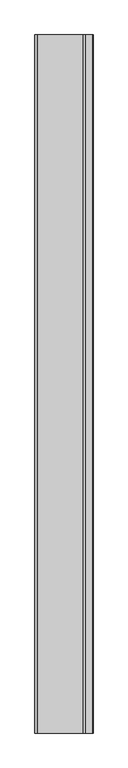
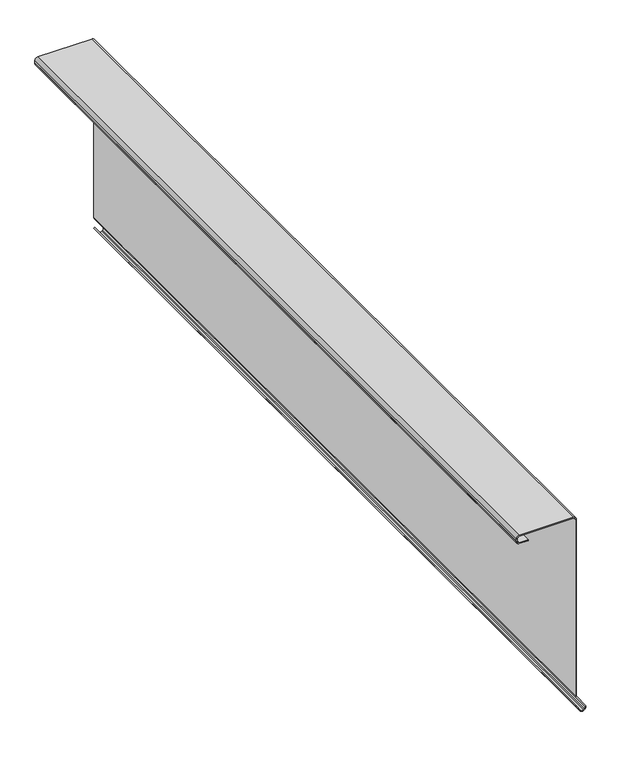
"""IFC4 building model written with IfcOpenShell, lengths in millimetres: proxy geometry, Flashing018 8742 : Flashing018 8742."""

from ifc_helpers import new_model, si_unit, point, frame, frame_2d, origin, place, context, project, spatial, polyline, circle_curve, trimmed, segment, composite_curve, outline, extrude, source, transform, mapped, element, save


def generic_models_9543aaf0(model_context):
    return source(origin(), model_context, "Body", "SweptSolid", [
        extrude(outline(composite_curve([segment(polyline([(43036.8907248, 17759.2743151), (43051.477598, 17749.0170677), (43050.3271805, 17747.3810543), (43035.7403074, 17757.6383018)]), True, "CONTINUOUS"), segment(trimmed(circle_curve(frame_2d((43039.8127852, 17763.429789)), 7.08), [point((43035.7403074, 17757.6383018))], [point((43034.0825771, 17767.5880476))], False, "CARTESIAN"), True, "CONTINUOUS"), segment(polyline([(43034.0825771, 17767.5880476), (43035.3752562, 17769.3693991)]), True, "CONTINUOUS"), segment(trimmed(circle_curve(frame_2d((43041.1054643, 17765.2111405)), 7.08), [point((43035.3752562, 17769.3693991))], [point((43045.1570771, 17771.0172436))], False, "CARTESIAN"), True, "CONTINUOUS"), segment(polyline([(43045.1570771, 17771.0172436), (43075.4099277, 17749.9062098)]), True, "CONTINUOUS"), segment(trimmed(circle_curve(frame_2d((43077.1724938, 17752.4320286)), 3.08), [point((43075.4099277, 17749.9062098))], [point((43077.1724938, 17749.3520286))], True, "CARTESIAN"), True, "CONTINUOUS"), segment(polyline([(43077.1724938, 17749.3520286), (43524.4015043, 17749.3520286)]), True, "CONTINUOUS"), segment(trimmed(circle_curve(frame_2d((43524.4015043, 17742.2720286)), 7.08), [point((43524.4015043, 17749.3520286))], [point((43531.4815043, 17742.2720286))], False, "CARTESIAN"), True, "CONTINUOUS"), segment(polyline([(43531.4815043, 17742.2720286), (43531.4815043, 17612.9320286)]), True, "CONTINUOUS"), segment(trimmed(circle_curve(frame_2d((43524.4015043, 17612.9320286)), 7.08), [point((43531.4815043, 17612.9320286))], [point((43524.4015043, 17605.8520286))], False, "CARTESIAN"), True, "CONTINUOUS"), segment(polyline([(43524.4015043, 17605.8520286), (43517.995098, 17605.8520286)]), True, "CONTINUOUS"), segment(trimmed(circle_curve(frame_2d((43517.995098, 17612.9320286)), 7.08), [point((43517.995098, 17605.8520286))], [point((43510.915098, 17612.9320286))], False, "CARTESIAN"), True, "CONTINUOUS"), segment(polyline([(43510.915098, 17612.9320286), (43510.915098, 17634.2284935), (43512.915098, 17634.2284935), (43512.915098, 17612.9320286)]), True, "CONTINUOUS"), segment(trimmed(circle_curve(frame_2d((43517.995098, 17612.9320286)), 5.08), [point((43512.915098, 17612.9320286))], [point((43517.995098, 17607.8520286))], True, "CARTESIAN"), True, "CONTINUOUS"), segment(polyline([(43517.995098, 17607.8520286), (43524.4015043, 17607.8520286)]), True, "CONTINUOUS"), segment(trimmed(circle_curve(frame_2d((43524.4015043, 17612.9320286)), 5.08), [point((43524.4015043, 17607.8520286))], [point((43529.4815043, 17612.9320286))], True, "CARTESIAN"), True, "CONTINUOUS"), segment(polyline([(43529.4815043, 17612.9320286), (43529.4815043, 17742.2720286)]), True, "CONTINUOUS"), segment(trimmed(circle_curve(frame_2d((43524.4015043, 17742.2720286)), 5.08), [point((43529.4815043, 17742.2720286))], [point((43524.4015043, 17747.3520286))], True, "CARTESIAN"), True, "CONTINUOUS"), segment(polyline([(43524.4015043, 17747.3520286), (43077.1724938, 17747.3520286)]), True, "CONTINUOUS"), segment(trimmed(circle_curve(frame_2d((43077.1724938, 17752.4320286)), 5.08), [point((43077.1724938, 17747.3520286))], [point((43074.2654043, 17748.2660676))], False, "CARTESIAN"), True, "CONTINUOUS"), segment(polyline([(43074.2654043, 17748.2660676), (43044.0125537, 17769.3771014)]), True, "CONTINUOUS"), segment(trimmed(circle_curve(frame_2d((43041.1054643, 17765.2111405)), 5.08), [point((43044.0125537, 17769.3771014))], [point((43036.993959, 17768.1947498))], True, "CARTESIAN"), True, "CONTINUOUS"), segment(polyline([(43036.993959, 17768.1947498), (43035.7012799, 17766.4133983)]), True, "CONTINUOUS"), segment(trimmed(circle_curve(frame_2d((43039.8127852, 17763.429789)), 5.08), [point((43035.7012799, 17766.4133983))], [point((43036.8907248, 17759.2743151))], True, "CARTESIAN"), True, "CONTINUOUS")], self_intersect=False)), frame((0.0, 7982.1507711, 0.0), z_axis=(0.0, 1.0, 0.0), x_axis=(0.0, 0.0, 1.0)), (0.0, 0.0, 1.0), 2000.0),
    ])


if __name__ == "__main__":
    model = new_model("IFC4")
    model_context = context("Model", 3, world=origin())
    ifc_project = project(units=[si_unit("LENGTHUNIT", "METRE", prefix="MILLI")], contexts=[model_context])
    site = spatial("IfcSite", under=ifc_project)
    building = spatial("IfcBuilding", under=site)
    placement = place(None, origin())
    generic_models_shape = generic_models_9543aaf0(model_context)
    element("IfcBuildingElementProxy", 1, Name="Flashing018 8742 : Flashing018 8742", ObjectType="Flashing018 8742 : Flashing018 8742", at=placement, inside=building, context=model_context, shape_type="MappedRepresentation", body=[
        mapped(generic_models_shape, transform((0.0, 0.0, 0.0), x_axis=(1.0, 0.0, 0.0), y_axis=(0.0, 1.0, 0.0), z_axis=(0.0, 0.0, 1.0))),
    ])
    save(model, "model.ifc")

# Revit data of these elements
# Type "Flashing018 8742 : Flashing018 8742"
#   NameOverride = "Flashing018"
# Element 1 (IfcBuildingElementProxy, "Flashing018 8742 : Flashing018 8742")
#   Materials on its faces: "HIGH EAVE FLASHING"
# Materials
#   "HIGH EAVE FLASHING": class "Unassigned", colour RGB 128 128 128, transparency 0
